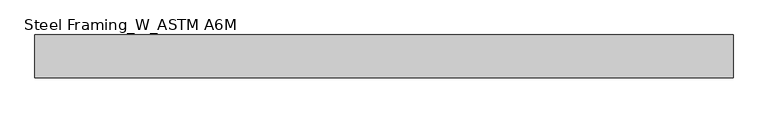
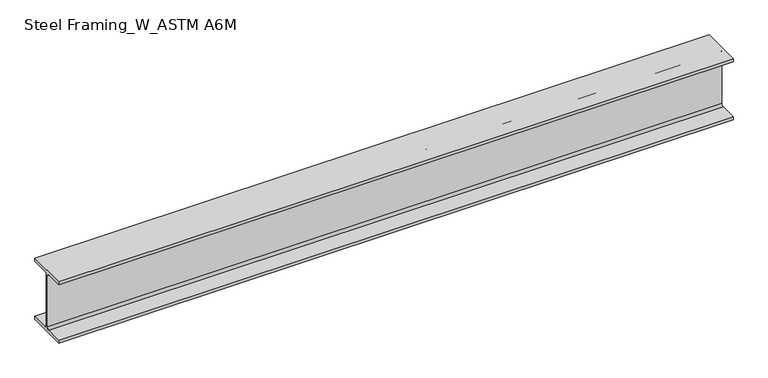
"""IFC4 building model written with IfcOpenShell, lengths in millimetres: beam geometry, Steel Framing_W_ASTM A6M : H_SB_AR_S02_W200x31.3_B6."""

import ifcopenshell
import ifcopenshell.guid

model = None  # the IFC model being written
_history = None  # IfcOwnerHistory: only IFC2X3 demands one
_inside = {}  # id of a spatial element -> (the spatial element, [elements in it])
_under = {}  # id of a project, library or spatial element -> (it, [spatial elements below it])
_declared = {}  # id of a project -> (the project, [libraries it declares])
_typed = {}  # id of a type object -> (the type object, [elements of that type])
_made_of = {}  # id of a material, layer set ... -> (it, [elements and type objects made of it])


def new_model(schema):
    """Start an empty IFC model of exactly this schema.

    Asked for "IFC4X3", IfcOpenShell would pick the latest addendum, in which some entities
    have other attributes; the version numbers below select the first issue.
    IFC2X3 requires an IfcOwnerHistory on every rooted entity: one is made here for all.
    """
    global model, _history
    if schema == "IFC4X3":
        model = ifcopenshell.file(schema_version=(4, 3, 0, 0))
    else:
        model = ifcopenshell.file(schema=schema)
    _inside.clear()
    _under.clear()
    _declared.clear()
    _typed.clear()
    _made_of.clear()
    _history = None
    if model.schema == "IFC2X3":
        org = make("IfcOrganization", Name="unknown")
        user = make(
            "IfcPersonAndOrganization",
            ThePerson=make("IfcPerson", FamilyName="unknown"),
            TheOrganization=org,
        )
        app = make(
            "IfcApplication",
            ApplicationDeveloper=org,
            Version="unknown",
            ApplicationFullName="unknown",
            ApplicationIdentifier="unknown",
        )
        _history = make(
            "IfcOwnerHistory",
            OwningUser=user,
            OwningApplication=app,
            ChangeAction="ADDED",
            CreationDate=0,
        )
    return model


def make(cls, **values):
    """One entity of the class cls with the attributes given. An attribute that is None is left unset."""
    return model.create_entity(
        cls, **{name: value for name, value in values.items() if value is not None}
    )


def rooted(cls, **values):
    """An entity with a GlobalId (a new one), such as an element, a storey or a relation."""
    return make(cls, GlobalId=ifcopenshell.guid.new(), OwnerHistory=_history, **values)


def si_unit(unit_type, name, prefix=None):
    """IfcSIUnit, for example si_unit("LENGTHUNIT", "METRE", prefix="MILLI")."""
    return make("IfcSIUnit", UnitType=unit_type, Prefix=prefix, Name=name)


def assignment(units):
    """IfcUnitAssignment: the units of a project."""
    return None if units is None else make("IfcUnitAssignment", Units=units)


def point(xyz):
    """IfcCartesianPoint."""
    return None if xyz is None else make("IfcCartesianPoint", Coordinates=xyz)


def direction(xyz):
    """IfcDirection."""
    return None if xyz is None else make("IfcDirection", DirectionRatios=xyz)


def frame(location, z_axis=None, x_axis=None):
    """IfcAxis2Placement3D, a coordinate frame: its origin and axes. An axis left out is left unset."""
    return make(
        "IfcAxis2Placement3D",
        Location=point(location),
        Axis=direction(z_axis),
        RefDirection=direction(x_axis),
    )


def frame_2d(location, x_axis=None):
    """IfcAxis2Placement2D, a coordinate frame in the plane: its origin and x axis."""
    return make(
        "IfcAxis2Placement2D", Location=point(location), RefDirection=direction(x_axis)
    )


def origin():
    """The frame at (0, 0, 0) with its axes left unset."""
    return frame((0.0, 0.0, 0.0))


def place(relative_to, where):
    """IfcLocalPlacement: puts the frame where relative to a parent placement (None: the world)."""
    return make(
        "IfcLocalPlacement", PlacementRelTo=relative_to, RelativePlacement=where
    )


def context(
    kind, dimensions, precision=None, world=None, true_north=None, identifier=None
):
    """IfcGeometricRepresentationContext, for example the 3D "Model" context."""
    return make(
        "IfcGeometricRepresentationContext",
        ContextIdentifier=identifier,
        ContextType=kind,
        CoordinateSpaceDimension=dimensions,
        Precision=precision,
        WorldCoordinateSystem=world,
        TrueNorth=true_north,
    )


def project(units=None, contexts=None):
    """IfcProject with its units and contexts."""
    return rooted(
        "IfcProject",
        Name="project",
        RepresentationContexts=contexts,
        UnitsInContext=assignment(units),
    )


def spatial(cls, under=None, at=None, **own):
    """A site, building, storey or space (cls), placed at a placement, below another one or the project."""
    s = rooted(cls, ObjectPlacement=at, **own)
    if under is not None:
        _under.setdefault(under.id(), (under, []))[1].append(s)
    return s


def polyline(points):
    """IfcPolyline through the points."""
    return make("IfcPolyline", Points=[point(p) for p in points])


def circle_curve(where, radius):
    """IfcCircle in the frame where."""
    return make("IfcCircle", Position=where, Radius=radius)


def trimmed(basis, trim1, trim2, sense, master):
    """IfcTrimmedCurve: the piece of a basis curve between two trims."""
    return make(
        "IfcTrimmedCurve",
        BasisCurve=basis,
        Trim1=trim1,
        Trim2=trim2,
        SenseAgreement=sense,
        MasterRepresentation=master,
    )


def segment(curve, same_sense, transition):
    """IfcCompositeCurveSegment."""
    return make(
        "IfcCompositeCurveSegment",
        Transition=transition,
        SameSense=same_sense,
        ParentCurve=curve,
    )


def composite_curve(segments, self_intersect=None):
    """IfcCompositeCurve: segments joined end to end."""
    return make("IfcCompositeCurve", Segments=segments, SelfIntersect=self_intersect)


def outline(outer, holes=None, kind="AREA"):
    """IfcArbitraryClosedProfileDef: a profile drawn as a closed curve; with holes, ...WithVoids."""
    if holes is None:
        return make("IfcArbitraryClosedProfileDef", ProfileType=kind, OuterCurve=outer)
    return make(
        "IfcArbitraryProfileDefWithVoids",
        ProfileType=kind,
        OuterCurve=outer,
        InnerCurves=holes,
    )


def extrude(swept, where, along, depth):
    """IfcExtrudedAreaSolid: the profile swept, set in the frame where, extruded along a direction by depth."""
    return make(
        "IfcExtrudedAreaSolid",
        SweptArea=swept,
        Position=where,
        ExtrudedDirection=direction(along),
        Depth=depth,
    )


def shape(context_of_items, identifier, shape_type, items):
    """IfcShapeRepresentation: the items that make up one representation, for example the "Body"."""
    return make(
        "IfcShapeRepresentation",
        ContextOfItems=context_of_items,
        RepresentationIdentifier=identifier,
        RepresentationType=shape_type,
        Items=items,
    )


def source(mapping_origin, context_of_items, identifier, shape_type, items):
    """IfcRepresentationMap: a shape defined once, which mapped items show again and again."""
    return make(
        "IfcRepresentationMap",
        MappingOrigin=mapping_origin,
        MappedRepresentation=shape(context_of_items, identifier, shape_type, items),
    )


def transform(
    local_origin,
    x_axis=None,
    y_axis=None,
    z_axis=None,
    scale=None,
    scale2=None,
    scale3=None,
    uniform=True,
):
    """IfcCartesianTransformationOperator3D, or its non-uniform kind. x_axis, y_axis, z_axis: its Axis1, 2, 3."""
    if uniform:
        return make(
            "IfcCartesianTransformationOperator3D",
            Axis1=direction(x_axis),
            Axis2=direction(y_axis),
            LocalOrigin=point(local_origin),
            Scale=scale,
            Axis3=direction(z_axis),
        )
    return make(
        "IfcCartesianTransformationOperator3DnonUniform",
        Axis1=direction(x_axis),
        Axis2=direction(y_axis),
        LocalOrigin=point(local_origin),
        Scale=scale,
        Axis3=direction(z_axis),
        Scale2=scale2,
        Scale3=scale3,
    )


def mapped(mapping_source, mapping_target):
    """IfcMappedItem: shows the shape of a source again, moved by a transform."""
    return make(
        "IfcMappedItem", MappingSource=mapping_source, MappingTarget=mapping_target
    )


def made_of(thing, what):
    """Note that an element or type object is made of a material, layer set ...; save() writes the relation."""
    if what is not None:
        _made_of.setdefault(what.id(), (what, []))[1].append(thing)
    return thing


def element(
    cls,
    number,
    at=None,
    inside=None,
    cuts=None,
    type_object=None,
    material=None,
    context=None,
    identifier="Body",
    shape_type=None,
    held_by="IfcProductDefinitionShape",
    body=None,
    shapes=None,
    **own,
):
    """One element of the class cls, such as IfcWall. Its Tag is "e" and its number.

    at: its placement. inside: the storey or other place that contains it. cuts: it is an
    opening in that element (IfcRelVoidsElement). A single representation is given by context,
    identifier, shape_type and body (its items); several are given by shapes. held_by: the class
    of the entity that holds the representations. save() writes the other relations.
    """
    e = rooted(cls, Tag="e%d" % number, ObjectPlacement=at, **own)
    if body is not None:
        shapes = [shape(context, identifier, shape_type, body)]
    if shapes is not None:
        e.Representation = make(held_by, Representations=shapes)
    if inside is not None:
        _inside.setdefault(inside.id(), (inside, []))[1].append(e)
    if cuts is not None:
        rooted(
            "IfcRelVoidsElement", RelatingBuildingElement=cuts, RelatedOpeningElement=e
        )
    if type_object is not None:
        _typed.setdefault(type_object.id(), (type_object, []))[1].append(e)
    return made_of(e, material)


def aggregate(whole, parts):
    """IfcRelAggregates: a whole, such as a stair, and the parts it consists of."""
    return rooted("IfcRelAggregates", RelatingObject=whole, RelatedObjects=parts)


def save(model, path):
    """Write the relations noted so far, then the file.

    IfcRelAggregates (storeys below a building ...), IfcRelContainedInSpatialStructure (elements
    in a storey), IfcRelDefinesByType, IfcRelAssociatesMaterial and IfcRelDeclares: one each for
    every whole, place, type object, material and project.
    """
    for whole, parts in _under.values():
        aggregate(whole, parts)
    for where, things in _inside.values():
        rooted(
            "IfcRelContainedInSpatialStructure",
            RelatedElements=things,
            RelatingStructure=where,
        )
    for kind, things in _typed.values():
        rooted("IfcRelDefinesByType", RelatedObjects=things, RelatingType=kind)
    for what, things in _made_of.values():
        rooted("IfcRelAssociatesMaterial", RelatedObjects=things, RelatingMaterial=what)
    for by, libraries in _declared.values():
        rooted("IfcRelDeclares", RelatingContext=by, RelatedDefinitions=libraries)
    model.write(path)


def steel_framing_w_astm_a6m_1b426b15(model_context):
    return source(origin(), model_context, "Body", "SweptSolid", [
        extrude(outline(composite_curve([segment(polyline([(67.0, -94.8), (67.0, -105.0), (-67.0, -105.0), (-67.0, -94.8), (-10.775, -94.8)]), True, "CONTINUOUS"), segment(trimmed(circle_curve(frame_2d((-10.775, -87.2)), 7.6), [point((-10.775, -94.8))], [point((-3.175, -87.2))], True, "CARTESIAN"), True, "CONTINUOUS"), segment(polyline([(-3.175, -87.2), (-3.175, 87.2)]), True, "CONTINUOUS"), segment(trimmed(circle_curve(frame_2d((-10.775, 87.2)), 7.6), [point((-3.175, 87.2))], [point((-10.775, 94.8))], True, "CARTESIAN"), True, "CONTINUOUS"), segment(polyline([(-10.775, 94.8), (-67.0, 94.8), (-67.0, 105.0), (67.0, 105.0), (67.0, 94.8), (10.775, 94.8)]), True, "CONTINUOUS"), segment(trimmed(circle_curve(frame_2d((10.775, 87.2)), 7.6), [point((10.775, 94.8))], [point((3.175, 87.2))], True, "CARTESIAN"), True, "CONTINUOUS"), segment(polyline([(3.175, 87.2), (3.175, -87.2)]), True, "CONTINUOUS"), segment(trimmed(circle_curve(frame_2d((10.775, -87.2)), 7.6), [point((3.175, -87.2))], [point((10.775, -94.8))], True, "CARTESIAN"), True, "CONTINUOUS"), segment(polyline([(10.775, -94.8), (67.0, -94.8)]), True, "CONTINUOUS")], self_intersect=False)), frame((-1135.8, 0.0, 0.0), z_axis=(1.0, 0.0, 0.0), x_axis=(0.0, 1.0, 0.0)), (0.0, 0.0, 1.0), 2189.1),
    ])


if __name__ == "__main__":
    model = new_model("IFC4")
    model_context = context("Model", 3, world=origin())
    ifc_project = project(units=[si_unit("LENGTHUNIT", "METRE", prefix="MILLI")], contexts=[model_context])
    site = spatial("IfcSite", under=ifc_project)
    building = spatial("IfcBuilding", under=site)
    placement = place(None, origin())
    steel_framing_w_astm_a6m_shape = steel_framing_w_astm_a6m_1b426b15(model_context)
    element("IfcBeam", 1, ObjectType="Steel Framing_W_ASTM A6M : H_SB_AR_S02_W200x31.3_B6", at=placement, inside=building, context=model_context, shape_type="MappedRepresentation", body=[
        mapped(steel_framing_w_astm_a6m_shape, transform((0.0, 0.0, 0.0), x_axis=(1.0, 0.0, 0.0), y_axis=(0.0, 1.0, 0.0), z_axis=(0.0, 0.0, 1.0))),
    ])
    save(model, "model.ifc")

# Revit data of these elements
# Type "Steel Framing_W_ASTM A6M : H_SB_AR_S02_W200x31.3_B6"
#   Type Mark = "B6"
#   Section Name Key = "W8x21"
#   Width = 13.4 cm
#   Web Thickness = 0.635 cm
#   Web Fillet = 0.76 cm
#   Warping Constant = 40800.0 cm⁶
#   Torsional Moment of Inertia = 11.70 cm⁴
#   Section Area = 39.7 cm²
#   Plastic Modulus weak axis = 93.2 cm³
#   Plastic Modulus strong axis = 334.0 cm³
#   Perimeter = 0.93 m²/m
#   Nominal Weight = 31.30 kgf/m
#   Moment of Inertia weak axis = 407.00 cm⁴
#   Moment of Inertia strong axis = 3130.00 cm⁴
#   Height = 21.0 cm
#   Flange Thickness = 1.02 cm
#   Elastic Modulus weak axis = 60.8 cm³
#   Elastic Modulus strong axis = 298.0 cm³
#   Centroid Vertical = 10.5 cm
#   Centroid Horizontal = 6.7 cm
#   Length [instance default] = 1500 mm
#   Structural Material [instance default] = Steel, 45-345
#   Bolt Spacing = 0
#   Assembly Code = ""
# Element 1 (IfcBeam, "Steel Framing_W_ASTM A6M : H_SB_AR_S02_W200x31.3_B6")
#   Materials on its faces: "Steel, 45-345"
# Materials
#   "Steel, 45-345": class "Metal", colour RGB 189 187 185, transparency 0, Description = "Steel 345 MPa", Cost = 0
